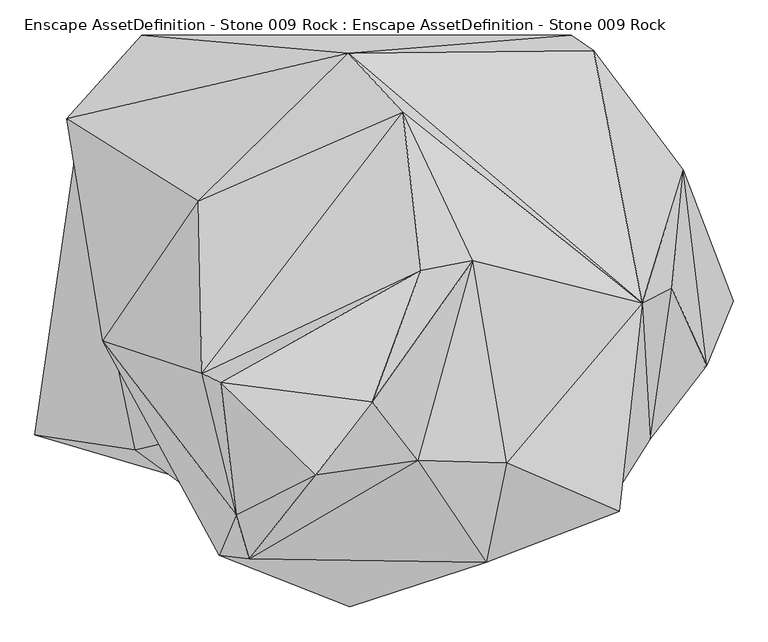
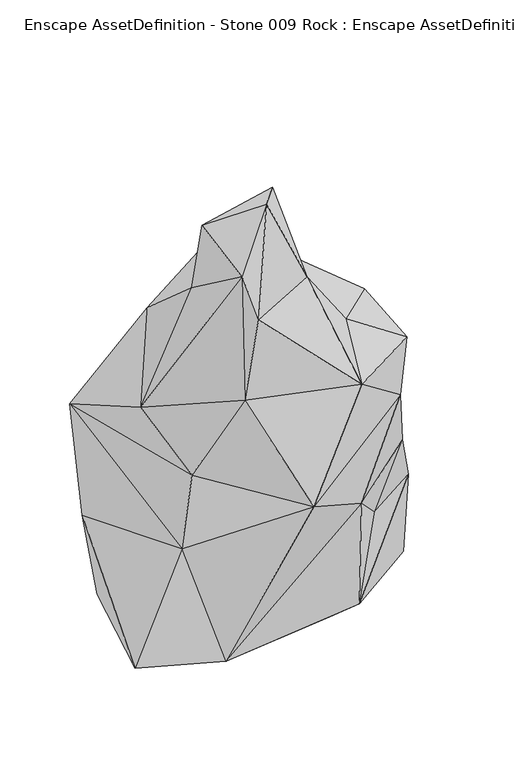
"""IFC4 building model written with IfcOpenShell, lengths in millimetres: geographic element geometry, Enscape AssetDefinition - Stone 009 Rock : Enscape AssetDefinition - Stone 009 Rock."""

import ifcopenshell
import ifcopenshell.guid

model = None  # the IFC model being written
_history = None  # IfcOwnerHistory: only IFC2X3 demands one
_inside = {}  # id of a spatial element -> (the spatial element, [elements in it])
_under = {}  # id of a project, library or spatial element -> (it, [spatial elements below it])
_declared = {}  # id of a project -> (the project, [libraries it declares])
_typed = {}  # id of a type object -> (the type object, [elements of that type])
_made_of = {}  # id of a material, layer set ... -> (it, [elements and type objects made of it])


def new_model(schema):
    """Start an empty IFC model of exactly this schema.

    Asked for "IFC4X3", IfcOpenShell would pick the latest addendum, in which some entities
    have other attributes; the version numbers below select the first issue.
    IFC2X3 requires an IfcOwnerHistory on every rooted entity: one is made here for all.
    """
    global model, _history
    if schema == "IFC4X3":
        model = ifcopenshell.file(schema_version=(4, 3, 0, 0))
    else:
        model = ifcopenshell.file(schema=schema)
    _inside.clear()
    _under.clear()
    _declared.clear()
    _typed.clear()
    _made_of.clear()
    _history = None
    if model.schema == "IFC2X3":
        org = make("IfcOrganization", Name="unknown")
        user = make(
            "IfcPersonAndOrganization",
            ThePerson=make("IfcPerson", FamilyName="unknown"),
            TheOrganization=org,
        )
        app = make(
            "IfcApplication",
            ApplicationDeveloper=org,
            Version="unknown",
            ApplicationFullName="unknown",
            ApplicationIdentifier="unknown",
        )
        _history = make(
            "IfcOwnerHistory",
            OwningUser=user,
            OwningApplication=app,
            ChangeAction="ADDED",
            CreationDate=0,
        )
    return model


def make(cls, **values):
    """One entity of the class cls with the attributes given. An attribute that is None is left unset."""
    return model.create_entity(
        cls, **{name: value for name, value in values.items() if value is not None}
    )


def rooted(cls, **values):
    """An entity with a GlobalId (a new one), such as an element, a storey or a relation."""
    return make(cls, GlobalId=ifcopenshell.guid.new(), OwnerHistory=_history, **values)


def si_unit(unit_type, name, prefix=None):
    """IfcSIUnit, for example si_unit("LENGTHUNIT", "METRE", prefix="MILLI")."""
    return make("IfcSIUnit", UnitType=unit_type, Prefix=prefix, Name=name)


def assignment(units):
    """IfcUnitAssignment: the units of a project."""
    return None if units is None else make("IfcUnitAssignment", Units=units)


def point(xyz):
    """IfcCartesianPoint."""
    return None if xyz is None else make("IfcCartesianPoint", Coordinates=xyz)


def direction(xyz):
    """IfcDirection."""
    return None if xyz is None else make("IfcDirection", DirectionRatios=xyz)


def frame(location, z_axis=None, x_axis=None):
    """IfcAxis2Placement3D, a coordinate frame: its origin and axes. An axis left out is left unset."""
    return make(
        "IfcAxis2Placement3D",
        Location=point(location),
        Axis=direction(z_axis),
        RefDirection=direction(x_axis),
    )


def origin():
    """The frame at (0, 0, 0) with its axes left unset."""
    return frame((0.0, 0.0, 0.0))


def place(relative_to, where):
    """IfcLocalPlacement: puts the frame where relative to a parent placement (None: the world)."""
    return make(
        "IfcLocalPlacement", PlacementRelTo=relative_to, RelativePlacement=where
    )


def context(
    kind, dimensions, precision=None, world=None, true_north=None, identifier=None
):
    """IfcGeometricRepresentationContext, for example the 3D "Model" context."""
    return make(
        "IfcGeometricRepresentationContext",
        ContextIdentifier=identifier,
        ContextType=kind,
        CoordinateSpaceDimension=dimensions,
        Precision=precision,
        WorldCoordinateSystem=world,
        TrueNorth=true_north,
    )


def project(units=None, contexts=None):
    """IfcProject with its units and contexts."""
    return rooted(
        "IfcProject",
        Name="project",
        RepresentationContexts=contexts,
        UnitsInContext=assignment(units),
    )


def spatial(cls, under=None, at=None, **own):
    """A site, building, storey or space (cls), placed at a placement, below another one or the project."""
    s = rooted(cls, ObjectPlacement=at, **own)
    if under is not None:
        _under.setdefault(under.id(), (under, []))[1].append(s)
    return s


def faces_of(points, faces, orient=None, outer=None):
    """IfcFace entities. A face is a list of loops; a loop is a list of indices into points, from 0.

    orient and outer hold one flag for each loop. By default every Orientation is true, the
    first loop of a face is its IfcFaceOuterBound and the others are IfcFaceBound.
    """
    made = []
    for i, loops in enumerate(faces):
        bounds = []
        for j, loop in enumerate(loops):
            is_outer = j == 0 if outer is None else outer[i][j]
            bounds.append(
                make(
                    "IfcFaceOuterBound" if is_outer else "IfcFaceBound",
                    Bound=make("IfcPolyLoop", Polygon=[points[k] for k in loop]),
                    Orientation=True if orient is None else orient[i][j],
                )
            )
        made.append(make("IfcFace", Bounds=bounds))
    return made


def faceted_brep(points, faces, orient=None, outer=None, voids=None):
    """IfcFacetedBrep: a solid bounded by flat faces; with voids (closed shells), ...WithVoids."""
    shared = [point(p) for p in points]
    hull = make("IfcClosedShell", CfsFaces=faces_of(shared, faces, orient, outer))
    if voids is None:
        return make("IfcFacetedBrep", Outer=hull)
    return make(
        "IfcFacetedBrepWithVoids",
        Outer=hull,
        Voids=[
            make(cls, CfsFaces=faces_of(shared, fs, o, b)) for cls, fs, o, b in voids
        ],
    )


def shape(context_of_items, identifier, shape_type, items):
    """IfcShapeRepresentation: the items that make up one representation, for example the "Body"."""
    return make(
        "IfcShapeRepresentation",
        ContextOfItems=context_of_items,
        RepresentationIdentifier=identifier,
        RepresentationType=shape_type,
        Items=items,
    )


def source(mapping_origin, context_of_items, identifier, shape_type, items):
    """IfcRepresentationMap: a shape defined once, which mapped items show again and again."""
    return make(
        "IfcRepresentationMap",
        MappingOrigin=mapping_origin,
        MappedRepresentation=shape(context_of_items, identifier, shape_type, items),
    )


def transform(
    local_origin,
    x_axis=None,
    y_axis=None,
    z_axis=None,
    scale=None,
    scale2=None,
    scale3=None,
    uniform=True,
):
    """IfcCartesianTransformationOperator3D, or its non-uniform kind. x_axis, y_axis, z_axis: its Axis1, 2, 3."""
    if uniform:
        return make(
            "IfcCartesianTransformationOperator3D",
            Axis1=direction(x_axis),
            Axis2=direction(y_axis),
            LocalOrigin=point(local_origin),
            Scale=scale,
            Axis3=direction(z_axis),
        )
    return make(
        "IfcCartesianTransformationOperator3DnonUniform",
        Axis1=direction(x_axis),
        Axis2=direction(y_axis),
        LocalOrigin=point(local_origin),
        Scale=scale,
        Axis3=direction(z_axis),
        Scale2=scale2,
        Scale3=scale3,
    )


def mapped(mapping_source, mapping_target):
    """IfcMappedItem: shows the shape of a source again, moved by a transform."""
    return make(
        "IfcMappedItem", MappingSource=mapping_source, MappingTarget=mapping_target
    )


def made_of(thing, what):
    """Note that an element or type object is made of a material, layer set ...; save() writes the relation."""
    if what is not None:
        _made_of.setdefault(what.id(), (what, []))[1].append(thing)
    return thing


def element(
    cls,
    number,
    at=None,
    inside=None,
    cuts=None,
    type_object=None,
    material=None,
    context=None,
    identifier="Body",
    shape_type=None,
    held_by="IfcProductDefinitionShape",
    body=None,
    shapes=None,
    **own,
):
    """One element of the class cls, such as IfcWall. Its Tag is "e" and its number.

    at: its placement. inside: the storey or other place that contains it. cuts: it is an
    opening in that element (IfcRelVoidsElement). A single representation is given by context,
    identifier, shape_type and body (its items); several are given by shapes. held_by: the class
    of the entity that holds the representations. save() writes the other relations.
    """
    e = rooted(cls, Tag="e%d" % number, ObjectPlacement=at, **own)
    if body is not None:
        shapes = [shape(context, identifier, shape_type, body)]
    if shapes is not None:
        e.Representation = make(held_by, Representations=shapes)
    if inside is not None:
        _inside.setdefault(inside.id(), (inside, []))[1].append(e)
    if cuts is not None:
        rooted(
            "IfcRelVoidsElement", RelatingBuildingElement=cuts, RelatedOpeningElement=e
        )
    if type_object is not None:
        _typed.setdefault(type_object.id(), (type_object, []))[1].append(e)
    return made_of(e, material)


def aggregate(whole, parts):
    """IfcRelAggregates: a whole, such as a stair, and the parts it consists of."""
    return rooted("IfcRelAggregates", RelatingObject=whole, RelatedObjects=parts)


def save(model, path):
    """Write the relations noted so far, then the file.

    IfcRelAggregates (storeys below a building ...), IfcRelContainedInSpatialStructure (elements
    in a storey), IfcRelDefinesByType, IfcRelAssociatesMaterial and IfcRelDeclares: one each for
    every whole, place, type object, material and project.
    """
    for whole, parts in _under.values():
        aggregate(whole, parts)
    for where, things in _inside.values():
        rooted(
            "IfcRelContainedInSpatialStructure",
            RelatedElements=things,
            RelatingStructure=where,
        )
    for kind, things in _typed.values():
        rooted("IfcRelDefinesByType", RelatedObjects=things, RelatingType=kind)
    for what, things in _made_of.values():
        rooted("IfcRelAssociatesMaterial", RelatedObjects=things, RelatingMaterial=what)
    for by, libraries in _declared.values():
        rooted("IfcRelDeclares", RelatingContext=by, RelatedDefinitions=libraries)
    model.write(path)


def enscape_assetdefinition_stone_009_rock_enscape_b3bb2d2c(model_context):
    return source(origin(), model_context, "Body", "Brep", [
        faceted_brep([(133.1470013, -239.3739969, 1330.597043), (222.1059948, 86.0859975, 1203.5759687), (58.4979989, -144.0339983, 1655.6770802), (498.145014, 17.3959993, 1000.4440546), (108.2609966, 327.7499974, 1162.8530025), (277.3990035, -243.761003, 1116.0999537), (137.8969997, 69.9210018, 1404.6020508), (-33.0369994, -262.7080083, 1692.0170784), (-188.1680042, -112.1710017, 1571.1489916), (-218.8110054, -97.9280025, 1323.9120245), (19.8149998, 424.2910147, 965.5359983), (-224.2009938, 182.791993, 1077.0599842), (-379.8579872, -45.1049991, 873.5209703), (-162.9229933, -328.3970058, 1489.2289639), (-141.6600049, -400.0779986, 1353.8700342), (-189.9310052, -393.8910067, 1046.2239981), (-282.4200094, -211.4859968, 671.2030172), (-438.7840033, 317.6000118, 688.3190274), (-316.1439896, 453.572005, 367.7639961), (-424.3589938, 258.6320043, 276.1569917), (-327.1630108, -222.1679986, 401.9719958), (22.3900005, -477.7970016, 601.2110114), (244.3699986, -405.1100016, 965.7059908), (461.0109925, -322.6070106, 1029.0679932), (434.6860051, -325.25599, 808.382988), (271.4329958, -354.9759984, 453.3709884), (-197.9549974, -283.6380005, -53.5259992), (-490.4209971, -197.8770047, -31.1220009), (305.3910136, -282.0830047, -2.1889999), (250.3429949, -186.2269938, -93.1129977), (-367.9809868, -140.2450055, -76.9419968), (401.5789926, -213.6099935, 287.8130078), (511.334002, -203.9790004, 530.0710201), (646.1669803, 20.7490008, -97.1850008), (603.1489968, -84.8560035, 288.5299921), (-337.2069895, 174.9619991, -119.1409975), (188.9670044, 329.2930126, -92.588), (565.433979, 233.713001, 556.155026), (552.3440242, 214.4159973, 99.8969972), (546.4490056, 41.7860001, 736.9769812), (382.4720085, 453.794986, 477.8980017), (419.1559851, 427.7929962, 703.3280134), (96.1930007, 431.6230118, 23.4779995), (-361.856997, 271.2459862, -67.5119981)], [[[0, 1, 2]], [[1, 3, 4]], [[1, 5, 3]], [[1, 6, 2]], [[1, 0, 5]], [[6, 1, 4]], [[7, 2, 8]], [[2, 6, 8]], [[2, 7, 0]], [[4, 9, 6]], [[8, 6, 9]], [[10, 11, 4]], [[3, 10, 4]], [[9, 4, 11]], [[9, 12, 13]], [[8, 9, 13]], [[9, 11, 12]], [[7, 8, 13]], [[0, 7, 14]], [[14, 7, 13]], [[12, 15, 13]], [[14, 13, 15]], [[16, 12, 17]], [[12, 16, 15]], [[11, 17, 12]], [[11, 10, 17]], [[17, 18, 19]], [[17, 19, 20]], [[20, 16, 17]], [[17, 10, 18]], [[16, 21, 15]], [[21, 16, 20]], [[21, 22, 15]], [[14, 15, 22]], [[22, 0, 14]], [[22, 5, 0]], [[22, 23, 5]], [[21, 24, 22]], [[23, 22, 24]], [[21, 25, 24]], [[21, 20, 26]], [[25, 21, 26]], [[19, 27, 20]], [[27, 26, 20]], [[28, 26, 29]], [[26, 27, 30]], [[26, 28, 25]], [[26, 30, 29]], [[31, 32, 25]], [[31, 25, 28]], [[24, 25, 32]], [[29, 33, 28]], [[34, 28, 33]], [[31, 28, 34]], [[30, 33, 29]], [[30, 27, 35]], [[36, 30, 35]], [[33, 30, 36]], [[37, 33, 38]], [[37, 34, 33]], [[33, 36, 38]], [[34, 37, 39]], [[32, 34, 39]], [[34, 32, 31]], [[39, 37, 3]], [[40, 41, 37]], [[37, 38, 40]], [[37, 41, 3]], [[38, 36, 42]], [[38, 42, 40]], [[36, 43, 42]], [[43, 36, 35]], [[35, 27, 43]], [[19, 18, 43]], [[19, 43, 27]], [[18, 42, 43]], [[40, 42, 18]], [[40, 10, 41]], [[40, 18, 10]], [[10, 3, 41]], [[24, 3, 23]], [[32, 3, 24]], [[32, 39, 3]], [[3, 5, 23]]]),
    ])


if __name__ == "__main__":
    model = new_model("IFC4")
    model_context = context("Model", 3, world=origin())
    ifc_project = project(units=[si_unit("LENGTHUNIT", "METRE", prefix="MILLI")], contexts=[model_context])
    site = spatial("IfcSite", under=ifc_project)
    building = spatial("IfcBuilding", under=site)
    placement = place(None, origin())
    enscape_assetdefinition_stone_009_rock_enscape_shape = enscape_assetdefinition_stone_009_rock_enscape_b3bb2d2c(model_context)
    element("IfcGeographicElement", 1, ObjectType="Enscape AssetDefinition - Stone 009 Rock : Enscape AssetDefinition - Stone 009 Rock", at=placement, inside=building, context=model_context, shape_type="MappedRepresentation", body=[
        mapped(enscape_assetdefinition_stone_009_rock_enscape_shape, transform((0.0, 0.0, 0.0), x_axis=(1.0, 0.0, 0.0), y_axis=(0.0, 1.0, 0.0), z_axis=(0.0, 0.0, 1.0))),
    ])
    save(model, "model.ifc")

# Revit data of these elements
# Type "Enscape AssetDefinition - Stone 009 Rock : Enscape AssetDefinition - Stone 009 Rock"
#   EnscapeAssetSource = "REMOTE"
#   EnscapeAssetId = "b75333a0-b9ae-4542-8500-551a42475bd0"
#   Height = 1.692017 m
#   EnscapeNativeAssetHeight = 1.692017 m
#   Default Elevation = 0
